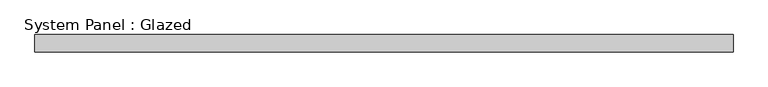
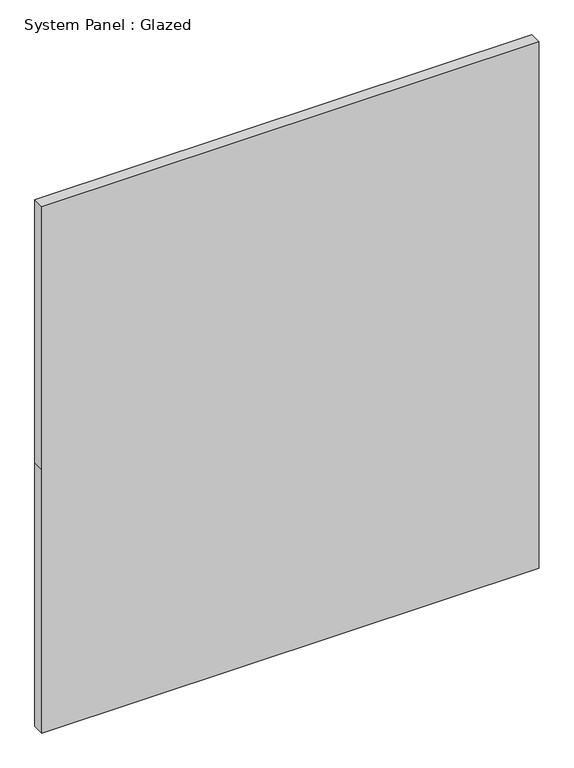
"""IFC4 building model written with IfcOpenShell, lengths in millimetres: plate geometry, System Panel : Glazed."""

import ifcopenshell
import ifcopenshell.guid

model = None  # the IFC model being written
_history = None  # IfcOwnerHistory: only IFC2X3 demands one
_inside = {}  # id of a spatial element -> (the spatial element, [elements in it])
_under = {}  # id of a project, library or spatial element -> (it, [spatial elements below it])
_declared = {}  # id of a project -> (the project, [libraries it declares])
_typed = {}  # id of a type object -> (the type object, [elements of that type])
_made_of = {}  # id of a material, layer set ... -> (it, [elements and type objects made of it])


def new_model(schema):
    """Start an empty IFC model of exactly this schema.

    Asked for "IFC4X3", IfcOpenShell would pick the latest addendum, in which some entities
    have other attributes; the version numbers below select the first issue.
    IFC2X3 requires an IfcOwnerHistory on every rooted entity: one is made here for all.
    """
    global model, _history
    if schema == "IFC4X3":
        model = ifcopenshell.file(schema_version=(4, 3, 0, 0))
    else:
        model = ifcopenshell.file(schema=schema)
    _inside.clear()
    _under.clear()
    _declared.clear()
    _typed.clear()
    _made_of.clear()
    _history = None
    if model.schema == "IFC2X3":
        org = make("IfcOrganization", Name="unknown")
        user = make(
            "IfcPersonAndOrganization",
            ThePerson=make("IfcPerson", FamilyName="unknown"),
            TheOrganization=org,
        )
        app = make(
            "IfcApplication",
            ApplicationDeveloper=org,
            Version="unknown",
            ApplicationFullName="unknown",
            ApplicationIdentifier="unknown",
        )
        _history = make(
            "IfcOwnerHistory",
            OwningUser=user,
            OwningApplication=app,
            ChangeAction="ADDED",
            CreationDate=0,
        )
    return model


def make(cls, **values):
    """One entity of the class cls with the attributes given. An attribute that is None is left unset."""
    return model.create_entity(
        cls, **{name: value for name, value in values.items() if value is not None}
    )


def rooted(cls, **values):
    """An entity with a GlobalId (a new one), such as an element, a storey or a relation."""
    return make(cls, GlobalId=ifcopenshell.guid.new(), OwnerHistory=_history, **values)


def si_unit(unit_type, name, prefix=None):
    """IfcSIUnit, for example si_unit("LENGTHUNIT", "METRE", prefix="MILLI")."""
    return make("IfcSIUnit", UnitType=unit_type, Prefix=prefix, Name=name)


def assignment(units):
    """IfcUnitAssignment: the units of a project."""
    return None if units is None else make("IfcUnitAssignment", Units=units)


def point(xyz):
    """IfcCartesianPoint."""
    return None if xyz is None else make("IfcCartesianPoint", Coordinates=xyz)


def direction(xyz):
    """IfcDirection."""
    return None if xyz is None else make("IfcDirection", DirectionRatios=xyz)


def frame(location, z_axis=None, x_axis=None):
    """IfcAxis2Placement3D, a coordinate frame: its origin and axes. An axis left out is left unset."""
    return make(
        "IfcAxis2Placement3D",
        Location=point(location),
        Axis=direction(z_axis),
        RefDirection=direction(x_axis),
    )


def origin():
    """The frame at (0, 0, 0) with its axes left unset."""
    return frame((0.0, 0.0, 0.0))


def place(relative_to, where):
    """IfcLocalPlacement: puts the frame where relative to a parent placement (None: the world)."""
    return make(
        "IfcLocalPlacement", PlacementRelTo=relative_to, RelativePlacement=where
    )


def context(
    kind, dimensions, precision=None, world=None, true_north=None, identifier=None
):
    """IfcGeometricRepresentationContext, for example the 3D "Model" context."""
    return make(
        "IfcGeometricRepresentationContext",
        ContextIdentifier=identifier,
        ContextType=kind,
        CoordinateSpaceDimension=dimensions,
        Precision=precision,
        WorldCoordinateSystem=world,
        TrueNorth=true_north,
    )


def project(units=None, contexts=None):
    """IfcProject with its units and contexts."""
    return rooted(
        "IfcProject",
        Name="project",
        RepresentationContexts=contexts,
        UnitsInContext=assignment(units),
    )


def spatial(cls, under=None, at=None, **own):
    """A site, building, storey or space (cls), placed at a placement, below another one or the project."""
    s = rooted(cls, ObjectPlacement=at, **own)
    if under is not None:
        _under.setdefault(under.id(), (under, []))[1].append(s)
    return s


def polyline(points):
    """IfcPolyline through the points."""
    return make("IfcPolyline", Points=[point(p) for p in points])


def outline(outer, holes=None, kind="AREA"):
    """IfcArbitraryClosedProfileDef: a profile drawn as a closed curve; with holes, ...WithVoids."""
    if holes is None:
        return make("IfcArbitraryClosedProfileDef", ProfileType=kind, OuterCurve=outer)
    return make(
        "IfcArbitraryProfileDefWithVoids",
        ProfileType=kind,
        OuterCurve=outer,
        InnerCurves=holes,
    )


def extrude(swept, where, along, depth):
    """IfcExtrudedAreaSolid: the profile swept, set in the frame where, extruded along a direction by depth."""
    return make(
        "IfcExtrudedAreaSolid",
        SweptArea=swept,
        Position=where,
        ExtrudedDirection=direction(along),
        Depth=depth,
    )


def shape(context_of_items, identifier, shape_type, items):
    """IfcShapeRepresentation: the items that make up one representation, for example the "Body"."""
    return make(
        "IfcShapeRepresentation",
        ContextOfItems=context_of_items,
        RepresentationIdentifier=identifier,
        RepresentationType=shape_type,
        Items=items,
    )


def source(mapping_origin, context_of_items, identifier, shape_type, items):
    """IfcRepresentationMap: a shape defined once, which mapped items show again and again."""
    return make(
        "IfcRepresentationMap",
        MappingOrigin=mapping_origin,
        MappedRepresentation=shape(context_of_items, identifier, shape_type, items),
    )


def transform(
    local_origin,
    x_axis=None,
    y_axis=None,
    z_axis=None,
    scale=None,
    scale2=None,
    scale3=None,
    uniform=True,
):
    """IfcCartesianTransformationOperator3D, or its non-uniform kind. x_axis, y_axis, z_axis: its Axis1, 2, 3."""
    if uniform:
        return make(
            "IfcCartesianTransformationOperator3D",
            Axis1=direction(x_axis),
            Axis2=direction(y_axis),
            LocalOrigin=point(local_origin),
            Scale=scale,
            Axis3=direction(z_axis),
        )
    return make(
        "IfcCartesianTransformationOperator3DnonUniform",
        Axis1=direction(x_axis),
        Axis2=direction(y_axis),
        LocalOrigin=point(local_origin),
        Scale=scale,
        Axis3=direction(z_axis),
        Scale2=scale2,
        Scale3=scale3,
    )


def mapped(mapping_source, mapping_target):
    """IfcMappedItem: shows the shape of a source again, moved by a transform."""
    return make(
        "IfcMappedItem", MappingSource=mapping_source, MappingTarget=mapping_target
    )


def made_of(thing, what):
    """Note that an element or type object is made of a material, layer set ...; save() writes the relation."""
    if what is not None:
        _made_of.setdefault(what.id(), (what, []))[1].append(thing)
    return thing


def element(
    cls,
    number,
    at=None,
    inside=None,
    cuts=None,
    type_object=None,
    material=None,
    context=None,
    identifier="Body",
    shape_type=None,
    held_by="IfcProductDefinitionShape",
    body=None,
    shapes=None,
    **own,
):
    """One element of the class cls, such as IfcWall. Its Tag is "e" and its number.

    at: its placement. inside: the storey or other place that contains it. cuts: it is an
    opening in that element (IfcRelVoidsElement). A single representation is given by context,
    identifier, shape_type and body (its items); several are given by shapes. held_by: the class
    of the entity that holds the representations. save() writes the other relations.
    """
    e = rooted(cls, Tag="e%d" % number, ObjectPlacement=at, **own)
    if body is not None:
        shapes = [shape(context, identifier, shape_type, body)]
    if shapes is not None:
        e.Representation = make(held_by, Representations=shapes)
    if inside is not None:
        _inside.setdefault(inside.id(), (inside, []))[1].append(e)
    if cuts is not None:
        rooted(
            "IfcRelVoidsElement", RelatingBuildingElement=cuts, RelatedOpeningElement=e
        )
    if type_object is not None:
        _typed.setdefault(type_object.id(), (type_object, []))[1].append(e)
    return made_of(e, material)


def aggregate(whole, parts):
    """IfcRelAggregates: a whole, such as a stair, and the parts it consists of."""
    return rooted("IfcRelAggregates", RelatingObject=whole, RelatedObjects=parts)


def save(model, path):
    """Write the relations noted so far, then the file.

    IfcRelAggregates (storeys below a building ...), IfcRelContainedInSpatialStructure (elements
    in a storey), IfcRelDefinesByType, IfcRelAssociatesMaterial and IfcRelDeclares: one each for
    every whole, place, type object, material and project.
    """
    for whole, parts in _under.values():
        aggregate(whole, parts)
    for where, things in _inside.values():
        rooted(
            "IfcRelContainedInSpatialStructure",
            RelatedElements=things,
            RelatingStructure=where,
        )
    for kind, things in _typed.values():
        rooted("IfcRelDefinesByType", RelatedObjects=things, RelatingType=kind)
    for what, things in _made_of.values():
        rooted("IfcRelAssociatesMaterial", RelatedObjects=things, RelatingMaterial=what)
    for by, libraries in _declared.values():
        rooted("IfcRelDeclares", RelatingContext=by, RelatedDefinitions=libraries)
    model.write(path)


def system_panel_glazed_abc00b7b(model_context):
    return source(origin(), model_context, "Body", "SweptSolid", [
        extrude(outline(polyline([(0.0, -516.255), (0.0, 516.255), (577.85, 516.255), (1155.7, 516.255), (1155.7, -516.255), (577.85, -516.255), (0.0, -516.255)])), frame((0.0, -44.45, 0.0), z_axis=(0.0, 1.0, 0.0), x_axis=(0.0, 0.0, 1.0)), (0.0, 0.0, 1.0), 25.4),
    ])


if __name__ == "__main__":
    model = new_model("IFC4")
    model_context = context("Model", 3, world=origin())
    ifc_project = project(units=[si_unit("LENGTHUNIT", "METRE", prefix="MILLI")], contexts=[model_context])
    site = spatial("IfcSite", under=ifc_project)
    building = spatial("IfcBuilding", under=site)
    placement = place(None, origin())
    system_panel_glazed_shape = system_panel_glazed_abc00b7b(model_context)
    element("IfcPlate", 1, ObjectType="System Panel : Glazed", at=placement, inside=building, context=model_context, shape_type="MappedRepresentation", body=[
        mapped(system_panel_glazed_shape, transform((0.0, 0.0, 0.0), x_axis=(1.0, 0.0, 0.0), y_axis=(0.0, 1.0, 0.0), z_axis=(0.0, 0.0, 1.0))),
    ])
    save(model, "model.ifc")

# Revit data of these elements
# Project information
#   SR Document GUID = "4c5931b3-dab8-40a9-800d-cf79e49c7e77"
# Element 1 (IfcPlate, "System Panel : Glazed")
#   Materials on its faces: "Glass"
# Materials
#   "Glass": class "Unassigned", colour RGB 0 0 255, transparency 0.75
